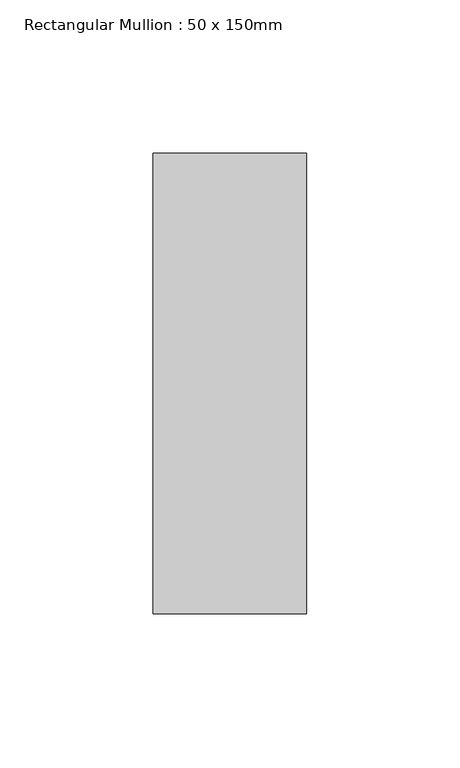
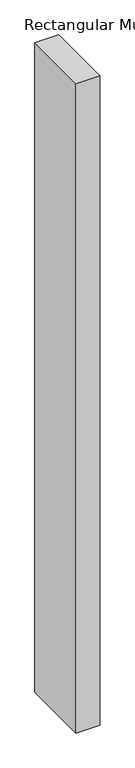
"""IFC4 building model written with IfcOpenShell, lengths in millimetres: member geometry, Rectangular Mullion : 50 x 150mm."""

from ifc_helpers import new_model, si_unit, frame, origin, place, context, project, spatial, polyline, outline, extrude, source, transform, mapped, element, save


def rectangular_mullion_50_x_150mm_f6f7edf2(model_context):
    return source(origin(), model_context, "Body", "SweptSolid", [
        extrude(outline(polyline([(25.0, 75.0), (25.0, -75.0), (-25.0, -75.0), (-25.0, 75.0), (25.0, 75.0)])), frame((0.0, 0.0, -1449.9999998), z_axis=(0.0, 0.0, 1.0), x_axis=(1.0, 0.0, 0.0)), (0.0, 0.0, 1.0), 1449.9999998),
    ])


if __name__ == "__main__":
    model = new_model("IFC4")
    model_context = context("Model", 3, world=origin())
    ifc_project = project(units=[si_unit("LENGTHUNIT", "METRE", prefix="MILLI")], contexts=[model_context])
    site = spatial("IfcSite", under=ifc_project)
    building = spatial("IfcBuilding", under=site)
    placement = place(None, origin())
    rectangular_mullion_50_x_150mm_shape = rectangular_mullion_50_x_150mm_f6f7edf2(model_context)
    element("IfcMember", 1, ObjectType="Rectangular Mullion : 50 x 150mm", at=placement, inside=building, context=model_context, shape_type="MappedRepresentation", body=[
        mapped(rectangular_mullion_50_x_150mm_shape, transform((0.0, 0.0, 0.0), x_axis=(1.0, 0.0, 0.0), y_axis=(0.0, 1.0, 0.0), z_axis=(0.0, 0.0, 1.0))),
    ])
    save(model, "model.ifc")

# Revit data of these elements
# Type "Rectangular Mullion : 50 x 150mm"
#   built-in parameter 1007304 = 0.492126 (stored number, unit not read)
#   built-in parameter 1007301 = 0.082021 (stored number, unit not read)
#   built-in parameter 1007300 = 0.082021 (stored number, unit not read)
# Element 1 (IfcMember, "Rectangular Mullion : 50 x 150mm")
#   Materials on its faces: "Aluminium"
# Materials
#   "Aluminium": class "Metal", colour RGB 247 247 247, transparency 0, Description = "Aluminium 6061", Cost = 0
